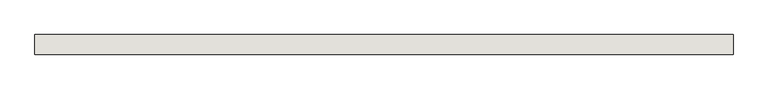
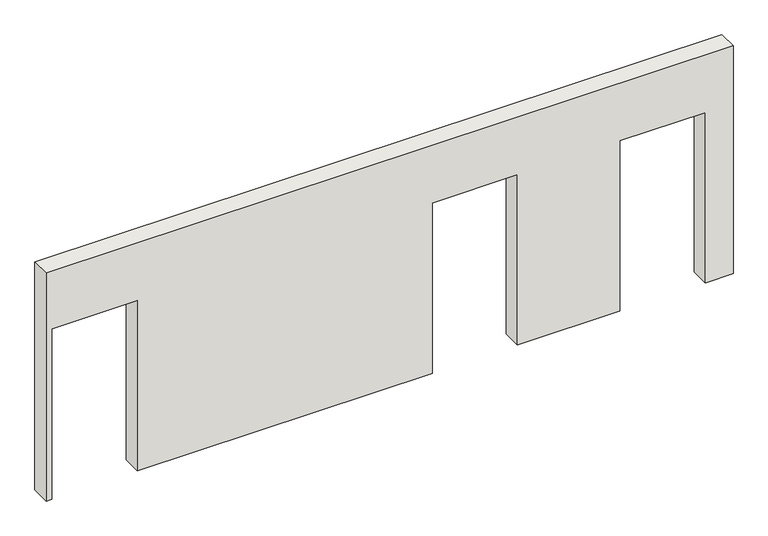
"""IFC4 building model written with IfcOpenShell, lengths in millimetres: wall geometry, Holzwand."""

import ifcopenshell
import ifcopenshell.guid

model = None  # the IFC model being written
_history = None  # IfcOwnerHistory: only IFC2X3 demands one
_inside = {}  # id of a spatial element -> (the spatial element, [elements in it])
_under = {}  # id of a project, library or spatial element -> (it, [spatial elements below it])
_declared = {}  # id of a project -> (the project, [libraries it declares])
_typed = {}  # id of a type object -> (the type object, [elements of that type])
_made_of = {}  # id of a material, layer set ... -> (it, [elements and type objects made of it])


def new_model(schema):
    """Start an empty IFC model of exactly this schema.

    Asked for "IFC4X3", IfcOpenShell would pick the latest addendum, in which some entities
    have other attributes; the version numbers below select the first issue.
    IFC2X3 requires an IfcOwnerHistory on every rooted entity: one is made here for all.
    """
    global model, _history
    if schema == "IFC4X3":
        model = ifcopenshell.file(schema_version=(4, 3, 0, 0))
    else:
        model = ifcopenshell.file(schema=schema)
    _inside.clear()
    _under.clear()
    _declared.clear()
    _typed.clear()
    _made_of.clear()
    _history = None
    if model.schema == "IFC2X3":
        org = make("IfcOrganization", Name="unknown")
        user = make(
            "IfcPersonAndOrganization",
            ThePerson=make("IfcPerson", FamilyName="unknown"),
            TheOrganization=org,
        )
        app = make(
            "IfcApplication",
            ApplicationDeveloper=org,
            Version="unknown",
            ApplicationFullName="unknown",
            ApplicationIdentifier="unknown",
        )
        _history = make(
            "IfcOwnerHistory",
            OwningUser=user,
            OwningApplication=app,
            ChangeAction="ADDED",
            CreationDate=0,
        )
    return model


def make(cls, **values):
    """One entity of the class cls with the attributes given. An attribute that is None is left unset."""
    return model.create_entity(
        cls, **{name: value for name, value in values.items() if value is not None}
    )


def rooted(cls, **values):
    """An entity with a GlobalId (a new one), such as an element, a storey or a relation."""
    return make(cls, GlobalId=ifcopenshell.guid.new(), OwnerHistory=_history, **values)


def si_unit(unit_type, name, prefix=None):
    """IfcSIUnit, for example si_unit("LENGTHUNIT", "METRE", prefix="MILLI")."""
    return make("IfcSIUnit", UnitType=unit_type, Prefix=prefix, Name=name)


def assignment(units):
    """IfcUnitAssignment: the units of a project."""
    return None if units is None else make("IfcUnitAssignment", Units=units)


def point(xyz):
    """IfcCartesianPoint."""
    return None if xyz is None else make("IfcCartesianPoint", Coordinates=xyz)


def direction(xyz):
    """IfcDirection."""
    return None if xyz is None else make("IfcDirection", DirectionRatios=xyz)


def frame(location, z_axis=None, x_axis=None):
    """IfcAxis2Placement3D, a coordinate frame: its origin and axes. An axis left out is left unset."""
    return make(
        "IfcAxis2Placement3D",
        Location=point(location),
        Axis=direction(z_axis),
        RefDirection=direction(x_axis),
    )


def origin():
    """The frame at (0, 0, 0) with its axes left unset."""
    return frame((0.0, 0.0, 0.0))


def place(relative_to, where):
    """IfcLocalPlacement: puts the frame where relative to a parent placement (None: the world)."""
    return make(
        "IfcLocalPlacement", PlacementRelTo=relative_to, RelativePlacement=where
    )


def context(
    kind, dimensions, precision=None, world=None, true_north=None, identifier=None
):
    """IfcGeometricRepresentationContext, for example the 3D "Model" context."""
    return make(
        "IfcGeometricRepresentationContext",
        ContextIdentifier=identifier,
        ContextType=kind,
        CoordinateSpaceDimension=dimensions,
        Precision=precision,
        WorldCoordinateSystem=world,
        TrueNorth=true_north,
    )


def project(units=None, contexts=None):
    """IfcProject with its units and contexts."""
    return rooted(
        "IfcProject",
        Name="project",
        RepresentationContexts=contexts,
        UnitsInContext=assignment(units),
    )


def spatial(cls, under=None, at=None, **own):
    """A site, building, storey or space (cls), placed at a placement, below another one or the project."""
    s = rooted(cls, ObjectPlacement=at, **own)
    if under is not None:
        _under.setdefault(under.id(), (under, []))[1].append(s)
    return s


def polyline(points):
    """IfcPolyline through the points."""
    return make("IfcPolyline", Points=[point(p) for p in points])


def outline(outer, holes=None, kind="AREA"):
    """IfcArbitraryClosedProfileDef: a profile drawn as a closed curve; with holes, ...WithVoids."""
    if holes is None:
        return make("IfcArbitraryClosedProfileDef", ProfileType=kind, OuterCurve=outer)
    return make(
        "IfcArbitraryProfileDefWithVoids",
        ProfileType=kind,
        OuterCurve=outer,
        InnerCurves=holes,
    )


def extrude(swept, where, along, depth):
    """IfcExtrudedAreaSolid: the profile swept, set in the frame where, extruded along a direction by depth."""
    return make(
        "IfcExtrudedAreaSolid",
        SweptArea=swept,
        Position=where,
        ExtrudedDirection=direction(along),
        Depth=depth,
    )


def shape(context_of_items, identifier, shape_type, items):
    """IfcShapeRepresentation: the items that make up one representation, for example the "Body"."""
    return make(
        "IfcShapeRepresentation",
        ContextOfItems=context_of_items,
        RepresentationIdentifier=identifier,
        RepresentationType=shape_type,
        Items=items,
    )


def source(mapping_origin, context_of_items, identifier, shape_type, items):
    """IfcRepresentationMap: a shape defined once, which mapped items show again and again."""
    return make(
        "IfcRepresentationMap",
        MappingOrigin=mapping_origin,
        MappedRepresentation=shape(context_of_items, identifier, shape_type, items),
    )


def transform(
    local_origin,
    x_axis=None,
    y_axis=None,
    z_axis=None,
    scale=None,
    scale2=None,
    scale3=None,
    uniform=True,
):
    """IfcCartesianTransformationOperator3D, or its non-uniform kind. x_axis, y_axis, z_axis: its Axis1, 2, 3."""
    if uniform:
        return make(
            "IfcCartesianTransformationOperator3D",
            Axis1=direction(x_axis),
            Axis2=direction(y_axis),
            LocalOrigin=point(local_origin),
            Scale=scale,
            Axis3=direction(z_axis),
        )
    return make(
        "IfcCartesianTransformationOperator3DnonUniform",
        Axis1=direction(x_axis),
        Axis2=direction(y_axis),
        LocalOrigin=point(local_origin),
        Scale=scale,
        Axis3=direction(z_axis),
        Scale2=scale2,
        Scale3=scale3,
    )


def mapped(mapping_source, mapping_target):
    """IfcMappedItem: shows the shape of a source again, moved by a transform."""
    return make(
        "IfcMappedItem", MappingSource=mapping_source, MappingTarget=mapping_target
    )


def made_of(thing, what):
    """Note that an element or type object is made of a material, layer set ...; save() writes the relation."""
    if what is not None:
        _made_of.setdefault(what.id(), (what, []))[1].append(thing)
    return thing


def element(
    cls,
    number,
    at=None,
    inside=None,
    cuts=None,
    type_object=None,
    material=None,
    context=None,
    identifier="Body",
    shape_type=None,
    held_by="IfcProductDefinitionShape",
    body=None,
    shapes=None,
    **own,
):
    """One element of the class cls, such as IfcWall. Its Tag is "e" and its number.

    at: its placement. inside: the storey or other place that contains it. cuts: it is an
    opening in that element (IfcRelVoidsElement). A single representation is given by context,
    identifier, shape_type and body (its items); several are given by shapes. held_by: the class
    of the entity that holds the representations. save() writes the other relations.
    """
    e = rooted(cls, Tag="e%d" % number, ObjectPlacement=at, **own)
    if body is not None:
        shapes = [shape(context, identifier, shape_type, body)]
    if shapes is not None:
        e.Representation = make(held_by, Representations=shapes)
    if inside is not None:
        _inside.setdefault(inside.id(), (inside, []))[1].append(e)
    if cuts is not None:
        rooted(
            "IfcRelVoidsElement", RelatingBuildingElement=cuts, RelatedOpeningElement=e
        )
    if type_object is not None:
        _typed.setdefault(type_object.id(), (type_object, []))[1].append(e)
    return made_of(e, material)


def aggregate(whole, parts):
    """IfcRelAggregates: a whole, such as a stair, and the parts it consists of."""
    return rooted("IfcRelAggregates", RelatingObject=whole, RelatedObjects=parts)


def save(model, path):
    """Write the relations noted so far, then the file.

    IfcRelAggregates (storeys below a building ...), IfcRelContainedInSpatialStructure (elements
    in a storey), IfcRelDefinesByType, IfcRelAssociatesMaterial and IfcRelDeclares: one each for
    every whole, place, type object, material and project.
    """
    for whole, parts in _under.values():
        aggregate(whole, parts)
    for where, things in _inside.values():
        rooted(
            "IfcRelContainedInSpatialStructure",
            RelatedElements=things,
            RelatingStructure=where,
        )
    for kind, things in _typed.values():
        rooted("IfcRelDefinesByType", RelatedObjects=things, RelatingType=kind)
    for what, things in _made_of.values():
        rooted("IfcRelAssociatesMaterial", RelatedObjects=things, RelatingMaterial=what)
    for by, libraries in _declared.values():
        rooted("IfcRelDeclares", RelatingContext=by, RelatedDefinitions=libraries)
    model.write(path)


def wall_67aac6ca(model_context):
    return source(origin(), model_context, "Body", "SweptSolid", [
        extrude(outline(polyline([(1870.0, 6837.13465), (0.0, 6837.13465), (0.0, 7125.0), (2500.0, 7125.0), (2500.0, 0.0), (0.0, 0.0), (0.0, 60.0), (1870.0, 60.0), (1870.0, 945.0), (0.0, 945.0), (0.0, 4003.8914512), (1870.0, 4003.8914512), (1870.0, 4888.8914512), (0.0, 4888.8914512), (0.0, 5952.13465), (1870.0, 5952.13465), (1870.0, 6837.13465)])), frame((0.0, 0.0, 0.0), z_axis=(0.0, 1.0, 0.0), x_axis=(0.0, 0.0, 1.0)), (0.0, 0.0, 1.0), 200.0),
    ])


if __name__ == "__main__":
    model = new_model("IFC4")
    model_context = context("Model", 3, world=origin())
    ifc_project = project(units=[si_unit("LENGTHUNIT", "METRE", prefix="MILLI")], contexts=[model_context])
    site = spatial("IfcSite", under=ifc_project)
    building = spatial("IfcBuilding", under=site)
    placement = place(None, origin())
    wall_shape = wall_67aac6ca(model_context)
    element("IfcWall", 1, ObjectType="Holzwand", at=placement, inside=building, context=model_context, shape_type="MappedRepresentation", body=[
        mapped(wall_shape, transform((0.0, 0.0, 0.0), x_axis=(1.0, 0.0, 0.0), y_axis=(0.0, 1.0, 0.0), z_axis=(0.0, 0.0, 1.0))),
    ])
    save(model, "model.ifc")

# Revit data of these elements
# Element 1 (IfcWall, "Holzwand")
#   Materials on its faces: "holzschalung"
# Materials
#   "holzschalung": class "Unassigned", colour RGB 128 128 128, transparency 0
